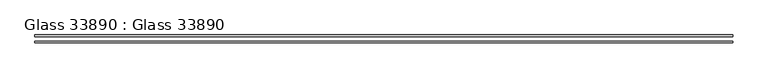
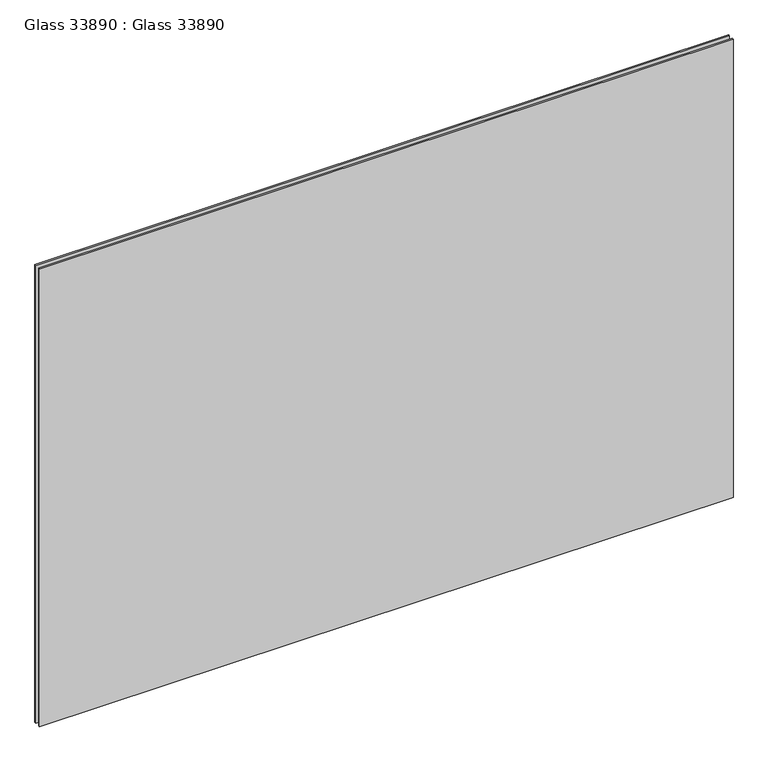
"""IFC4 building model written with IfcOpenShell, lengths in millimetres: proxy geometry, Glass 33890 : Glass 33890."""

from ifc_helpers import new_model, si_unit, frame, origin, place, context, project, spatial, polyline, outline, extrude, source, transform, mapped, element, save


def glass_33890_glass_33890_7f8999f5(model_context):
    return source(origin(), model_context, "Body", "SweptSolid", [
        extrude(outline(polyline([(14383.0178845, -4394.1834255), (14383.0178845, -4398.9459255), (12383.0178845, -4398.9459255), (12383.0178845, -4394.1834255), (14383.0178845, -4394.1834255)])), frame((0.0, 0.0, 41130.5392812), z_axis=(0.0, 0.0, 1.0), x_axis=(1.0, 0.0, 0.0)), (0.0, 0.0, 1.0), 1396.8024401),
        extrude(outline(polyline([(14383.0178845, -4412.1834255), (14383.0178845, -4416.9459255), (12383.0178845, -4416.9459255), (12383.0178845, -4412.1834255), (14383.0178845, -4412.1834255)])), frame((0.0, 0.0, 41130.5392812), z_axis=(0.0, 0.0, 1.0), x_axis=(1.0, 0.0, 0.0)), (0.0, 0.0, 1.0), 1396.8024401),
    ])


if __name__ == "__main__":
    model = new_model("IFC4")
    model_context = context("Model", 3, world=origin())
    ifc_project = project(units=[si_unit("LENGTHUNIT", "METRE", prefix="MILLI")], contexts=[model_context])
    site = spatial("IfcSite", under=ifc_project)
    building = spatial("IfcBuilding", under=site)
    placement = place(None, origin())
    glass_33890_glass_33890_shape = glass_33890_glass_33890_7f8999f5(model_context)
    element("IfcBuildingElementProxy", 1, Name="Glass 33890 : Glass 33890", ObjectType="Glass 33890 : Glass 33890", at=placement, inside=building, context=model_context, shape_type="MappedRepresentation", body=[
        mapped(glass_33890_glass_33890_shape, transform((0.0, 0.0, 0.0), x_axis=(1.0, 0.0, 0.0), y_axis=(0.0, 1.0, 0.0), z_axis=(0.0, 0.0, 1.0))),
    ])
    save(model, "model.ifc")

# Revit data of these elements
# Type "Glass 33890 : Glass 33890"
#   NameOverride = "Glass"
# Element 1 (IfcBuildingElementProxy, "Glass 33890 : Glass 33890")
#   Materials on its faces: "1\" INSULATED GLAZING"
# Materials
#   "1\" INSULATED GLAZING": class "Unassigned", colour RGB 146 199 212, transparency 0
